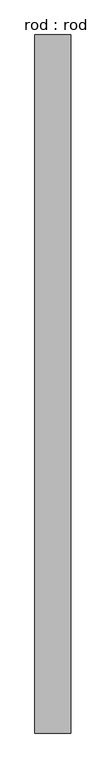
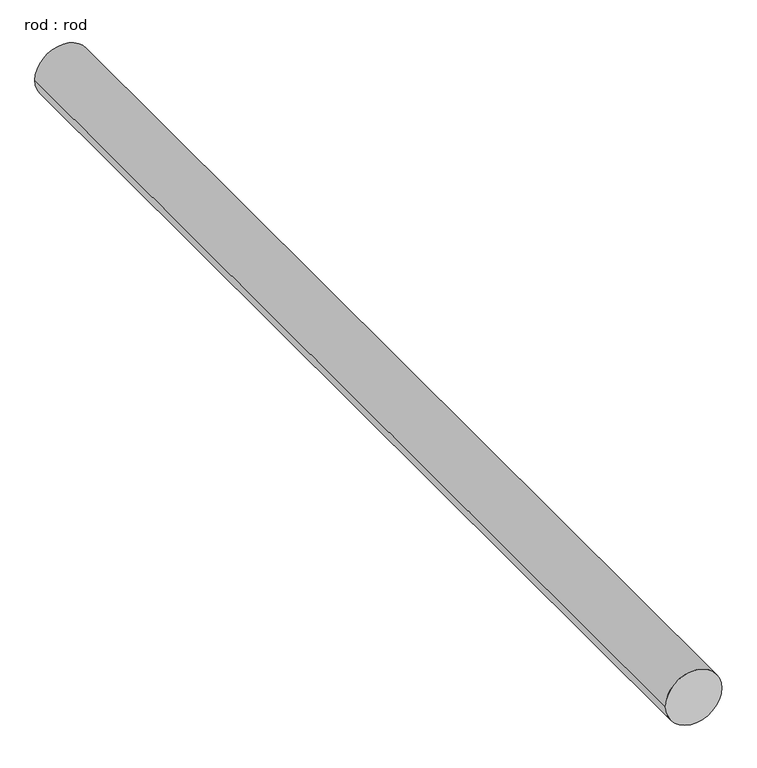
"""IFC4 building model written with IfcOpenShell, lengths in millimetres: proxy geometry, rod : rod."""

from ifc_helpers import new_model, si_unit, point, frame, frame_2d, origin, place, context, project, spatial, circle_curve, trimmed, segment, composite_curve, outline, extrude, source, transform, mapped, element, save


def rod_rod_892b5ed2(model_context):
    return source(origin(), model_context, "Body", "SweptSolid", [
        extrude(outline(composite_curve([segment(trimmed(circle_curve(frame_2d((0.0108462, 0.0)), 200.0), [point((0.0108462, 200.0))], [point((0.0108462, -200.0))], False, "CARTESIAN"), True, "CONTINUOUS"), segment(trimmed(circle_curve(frame_2d((0.0108462, 0.0)), 200.0), [point((0.0108462, -200.0))], [point((0.0108462, 200.0))], False, "CARTESIAN"), True, "CONTINUOUS")], self_intersect=False)), frame((0.0, 208.0225315, 0.0), z_axis=(0.0, 1.0, 0.0), x_axis=(0.0, 0.0, 1.0)), (0.0, 0.0, 1.0), 7769.4121677),
    ])


if __name__ == "__main__":
    model = new_model("IFC4")
    model_context = context("Model", 3, world=origin())
    ifc_project = project(units=[si_unit("LENGTHUNIT", "METRE", prefix="MILLI")], contexts=[model_context])
    site = spatial("IfcSite", under=ifc_project)
    building = spatial("IfcBuilding", under=site)
    placement = place(None, origin())
    rod_rod_shape = rod_rod_892b5ed2(model_context)
    element("IfcBuildingElementProxy", 1, Name="rod : rod", ObjectType="rod : rod", at=placement, inside=building, context=model_context, shape_type="MappedRepresentation", body=[
        mapped(rod_rod_shape, transform((0.0, 0.0, 0.0), x_axis=(1.0, 0.0, 0.0), y_axis=(0.0, 1.0, 0.0), z_axis=(0.0, 0.0, 1.0))),
    ])
    save(model, "model.ifc")

# Revit data of these elements
# Type "rod : rod"
#   Default Elevation = 0
